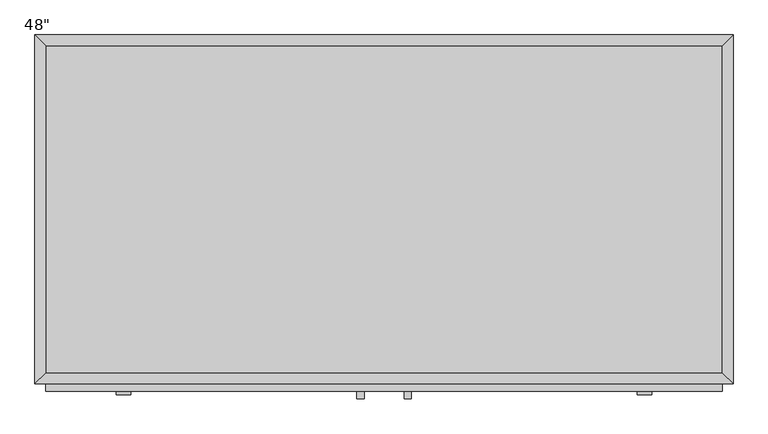
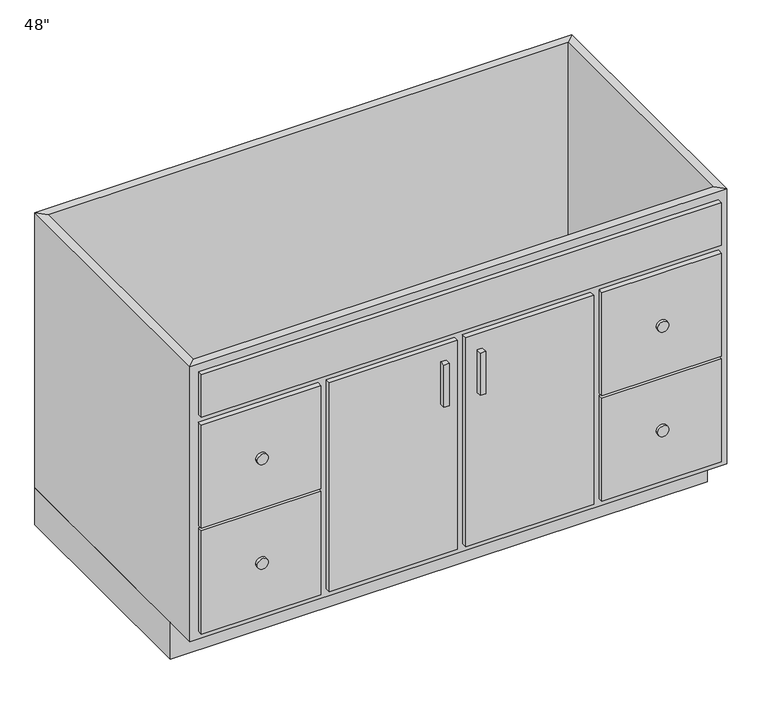
"""IFC4 building model written with IfcOpenShell, lengths in millimetres: furniture geometry."""

import ifcopenshell
import ifcopenshell.guid

model = None  # the IFC model being written
_history = None  # IfcOwnerHistory: only IFC2X3 demands one
_inside = {}  # id of a spatial element -> (the spatial element, [elements in it])
_under = {}  # id of a project, library or spatial element -> (it, [spatial elements below it])
_declared = {}  # id of a project -> (the project, [libraries it declares])
_typed = {}  # id of a type object -> (the type object, [elements of that type])
_made_of = {}  # id of a material, layer set ... -> (it, [elements and type objects made of it])


def new_model(schema):
    """Start an empty IFC model of exactly this schema.

    Asked for "IFC4X3", IfcOpenShell would pick the latest addendum, in which some entities
    have other attributes; the version numbers below select the first issue.
    IFC2X3 requires an IfcOwnerHistory on every rooted entity: one is made here for all.
    """
    global model, _history
    if schema == "IFC4X3":
        model = ifcopenshell.file(schema_version=(4, 3, 0, 0))
    else:
        model = ifcopenshell.file(schema=schema)
    _inside.clear()
    _under.clear()
    _declared.clear()
    _typed.clear()
    _made_of.clear()
    _history = None
    if model.schema == "IFC2X3":
        org = make("IfcOrganization", Name="unknown")
        user = make(
            "IfcPersonAndOrganization",
            ThePerson=make("IfcPerson", FamilyName="unknown"),
            TheOrganization=org,
        )
        app = make(
            "IfcApplication",
            ApplicationDeveloper=org,
            Version="unknown",
            ApplicationFullName="unknown",
            ApplicationIdentifier="unknown",
        )
        _history = make(
            "IfcOwnerHistory",
            OwningUser=user,
            OwningApplication=app,
            ChangeAction="ADDED",
            CreationDate=0,
        )
    return model


def make(cls, **values):
    """One entity of the class cls with the attributes given. An attribute that is None is left unset."""
    return model.create_entity(
        cls, **{name: value for name, value in values.items() if value is not None}
    )


def rooted(cls, **values):
    """An entity with a GlobalId (a new one), such as an element, a storey or a relation."""
    return make(cls, GlobalId=ifcopenshell.guid.new(), OwnerHistory=_history, **values)


def si_unit(unit_type, name, prefix=None):
    """IfcSIUnit, for example si_unit("LENGTHUNIT", "METRE", prefix="MILLI")."""
    return make("IfcSIUnit", UnitType=unit_type, Prefix=prefix, Name=name)


def assignment(units):
    """IfcUnitAssignment: the units of a project."""
    return None if units is None else make("IfcUnitAssignment", Units=units)


def point(xyz):
    """IfcCartesianPoint."""
    return None if xyz is None else make("IfcCartesianPoint", Coordinates=xyz)


def direction(xyz):
    """IfcDirection."""
    return None if xyz is None else make("IfcDirection", DirectionRatios=xyz)


def frame(location, z_axis=None, x_axis=None):
    """IfcAxis2Placement3D, a coordinate frame: its origin and axes. An axis left out is left unset."""
    return make(
        "IfcAxis2Placement3D",
        Location=point(location),
        Axis=direction(z_axis),
        RefDirection=direction(x_axis),
    )


def frame_2d(location, x_axis=None):
    """IfcAxis2Placement2D, a coordinate frame in the plane: its origin and x axis."""
    return make(
        "IfcAxis2Placement2D", Location=point(location), RefDirection=direction(x_axis)
    )


def origin():
    """The frame at (0, 0, 0) with its axes left unset."""
    return frame((0.0, 0.0, 0.0))


def origin_with_axes():
    """The frame at (0, 0, 0) with the z axis (0, 0, 1) and the x axis (1, 0, 0) written out."""
    return frame((0.0, 0.0, 0.0), z_axis=(0.0, 0.0, 1.0), x_axis=(1.0, 0.0, 0.0))


def place(relative_to, where):
    """IfcLocalPlacement: puts the frame where relative to a parent placement (None: the world)."""
    return make(
        "IfcLocalPlacement", PlacementRelTo=relative_to, RelativePlacement=where
    )


def context(
    kind, dimensions, precision=None, world=None, true_north=None, identifier=None
):
    """IfcGeometricRepresentationContext, for example the 3D "Model" context."""
    return make(
        "IfcGeometricRepresentationContext",
        ContextIdentifier=identifier,
        ContextType=kind,
        CoordinateSpaceDimension=dimensions,
        Precision=precision,
        WorldCoordinateSystem=world,
        TrueNorth=true_north,
    )


def project(units=None, contexts=None):
    """IfcProject with its units and contexts."""
    return rooted(
        "IfcProject",
        Name="project",
        RepresentationContexts=contexts,
        UnitsInContext=assignment(units),
    )


def spatial(cls, under=None, at=None, **own):
    """A site, building, storey or space (cls), placed at a placement, below another one or the project."""
    s = rooted(cls, ObjectPlacement=at, **own)
    if under is not None:
        _under.setdefault(under.id(), (under, []))[1].append(s)
    return s


def polyline(points):
    """IfcPolyline through the points."""
    return make("IfcPolyline", Points=[point(p) for p in points])


def circle_curve(where, radius):
    """IfcCircle in the frame where."""
    return make("IfcCircle", Position=where, Radius=radius)


def trimmed(basis, trim1, trim2, sense, master):
    """IfcTrimmedCurve: the piece of a basis curve between two trims."""
    return make(
        "IfcTrimmedCurve",
        BasisCurve=basis,
        Trim1=trim1,
        Trim2=trim2,
        SenseAgreement=sense,
        MasterRepresentation=master,
    )


def segment(curve, same_sense, transition):
    """IfcCompositeCurveSegment."""
    return make(
        "IfcCompositeCurveSegment",
        Transition=transition,
        SameSense=same_sense,
        ParentCurve=curve,
    )


def composite_curve(segments, self_intersect=None):
    """IfcCompositeCurve: segments joined end to end."""
    return make("IfcCompositeCurve", Segments=segments, SelfIntersect=self_intersect)


def outline(outer, holes=None, kind="AREA"):
    """IfcArbitraryClosedProfileDef: a profile drawn as a closed curve; with holes, ...WithVoids."""
    if holes is None:
        return make("IfcArbitraryClosedProfileDef", ProfileType=kind, OuterCurve=outer)
    return make(
        "IfcArbitraryProfileDefWithVoids",
        ProfileType=kind,
        OuterCurve=outer,
        InnerCurves=holes,
    )


def extrude(swept, where, along, depth):
    """IfcExtrudedAreaSolid: the profile swept, set in the frame where, extruded along a direction by depth."""
    return make(
        "IfcExtrudedAreaSolid",
        SweptArea=swept,
        Position=where,
        ExtrudedDirection=direction(along),
        Depth=depth,
    )


def faces_of(points, faces, orient=None, outer=None):
    """IfcFace entities. A face is a list of loops; a loop is a list of indices into points, from 0.

    orient and outer hold one flag for each loop. By default every Orientation is true, the
    first loop of a face is its IfcFaceOuterBound and the others are IfcFaceBound.
    """
    made = []
    for i, loops in enumerate(faces):
        bounds = []
        for j, loop in enumerate(loops):
            is_outer = j == 0 if outer is None else outer[i][j]
            bounds.append(
                make(
                    "IfcFaceOuterBound" if is_outer else "IfcFaceBound",
                    Bound=make("IfcPolyLoop", Polygon=[points[k] for k in loop]),
                    Orientation=True if orient is None else orient[i][j],
                )
            )
        made.append(make("IfcFace", Bounds=bounds))
    return made


def faceted_brep(points, faces, orient=None, outer=None, voids=None):
    """IfcFacetedBrep: a solid bounded by flat faces; with voids (closed shells), ...WithVoids."""
    shared = [point(p) for p in points]
    hull = make("IfcClosedShell", CfsFaces=faces_of(shared, faces, orient, outer))
    if voids is None:
        return make("IfcFacetedBrep", Outer=hull)
    return make(
        "IfcFacetedBrepWithVoids",
        Outer=hull,
        Voids=[
            make(cls, CfsFaces=faces_of(shared, fs, o, b)) for cls, fs, o, b in voids
        ],
    )


def shape(context_of_items, identifier, shape_type, items):
    """IfcShapeRepresentation: the items that make up one representation, for example the "Body"."""
    return make(
        "IfcShapeRepresentation",
        ContextOfItems=context_of_items,
        RepresentationIdentifier=identifier,
        RepresentationType=shape_type,
        Items=items,
    )


def source(mapping_origin, context_of_items, identifier, shape_type, items):
    """IfcRepresentationMap: a shape defined once, which mapped items show again and again."""
    return make(
        "IfcRepresentationMap",
        MappingOrigin=mapping_origin,
        MappedRepresentation=shape(context_of_items, identifier, shape_type, items),
    )


def transform(
    local_origin,
    x_axis=None,
    y_axis=None,
    z_axis=None,
    scale=None,
    scale2=None,
    scale3=None,
    uniform=True,
):
    """IfcCartesianTransformationOperator3D, or its non-uniform kind. x_axis, y_axis, z_axis: its Axis1, 2, 3."""
    if uniform:
        return make(
            "IfcCartesianTransformationOperator3D",
            Axis1=direction(x_axis),
            Axis2=direction(y_axis),
            LocalOrigin=point(local_origin),
            Scale=scale,
            Axis3=direction(z_axis),
        )
    return make(
        "IfcCartesianTransformationOperator3DnonUniform",
        Axis1=direction(x_axis),
        Axis2=direction(y_axis),
        LocalOrigin=point(local_origin),
        Scale=scale,
        Axis3=direction(z_axis),
        Scale2=scale2,
        Scale3=scale3,
    )


def mapped(mapping_source, mapping_target):
    """IfcMappedItem: shows the shape of a source again, moved by a transform."""
    return make(
        "IfcMappedItem", MappingSource=mapping_source, MappingTarget=mapping_target
    )


def made_of(thing, what):
    """Note that an element or type object is made of a material, layer set ...; save() writes the relation."""
    if what is not None:
        _made_of.setdefault(what.id(), (what, []))[1].append(thing)
    return thing


def element(
    cls,
    number,
    at=None,
    inside=None,
    cuts=None,
    type_object=None,
    material=None,
    context=None,
    identifier="Body",
    shape_type=None,
    held_by="IfcProductDefinitionShape",
    body=None,
    shapes=None,
    **own,
):
    """One element of the class cls, such as IfcWall. Its Tag is "e" and its number.

    at: its placement. inside: the storey or other place that contains it. cuts: it is an
    opening in that element (IfcRelVoidsElement). A single representation is given by context,
    identifier, shape_type and body (its items); several are given by shapes. held_by: the class
    of the entity that holds the representations. save() writes the other relations.
    """
    e = rooted(cls, Tag="e%d" % number, ObjectPlacement=at, **own)
    if body is not None:
        shapes = [shape(context, identifier, shape_type, body)]
    if shapes is not None:
        e.Representation = make(held_by, Representations=shapes)
    if inside is not None:
        _inside.setdefault(inside.id(), (inside, []))[1].append(e)
    if cuts is not None:
        rooted(
            "IfcRelVoidsElement", RelatingBuildingElement=cuts, RelatedOpeningElement=e
        )
    if type_object is not None:
        _typed.setdefault(type_object.id(), (type_object, []))[1].append(e)
    return made_of(e, material)


def aggregate(whole, parts):
    """IfcRelAggregates: a whole, such as a stair, and the parts it consists of."""
    return rooted("IfcRelAggregates", RelatingObject=whole, RelatedObjects=parts)


def save(model, path):
    """Write the relations noted so far, then the file.

    IfcRelAggregates (storeys below a building ...), IfcRelContainedInSpatialStructure (elements
    in a storey), IfcRelDefinesByType, IfcRelAssociatesMaterial and IfcRelDeclares: one each for
    every whole, place, type object, material and project.
    """
    for whole, parts in _under.values():
        aggregate(whole, parts)
    for where, things in _inside.values():
        rooted(
            "IfcRelContainedInSpatialStructure",
            RelatedElements=things,
            RelatingStructure=where,
        )
    for kind, things in _typed.values():
        rooted("IfcRelDefinesByType", RelatedObjects=things, RelatingType=kind)
    for what, things in _made_of.values():
        rooted("IfcRelAssociatesMaterial", RelatedObjects=things, RelatingMaterial=what)
    for by, libraries in _declared.values():
        rooted("IfcRelDeclares", RelatingContext=by, RelatedDefinitions=libraries)
    model.write(path)


def furniture_7e5e5cd5(model_context):
    return source(origin(), model_context, "Body", "SolidModel", [
        extrude(outline(polyline([(55.91996, -635.0), (43.21996, -635.0), (43.21996, -622.3), (55.91996, -622.3), (55.91996, -635.0)])), frame((0.0, 0.0, 469.9), z_axis=(0.0, 0.0, 1.0), x_axis=(1.0, 0.0, 0.0)), (0.0, 0.0, 1.0), 101.6),
        extrude(outline(polyline([(138.46996, -635.0), (125.76996, -635.0), (125.76996, -622.3), (138.46996, -622.3), (138.46996, -635.0)])), frame((0.0, 0.0, 469.9), z_axis=(0.0, 0.0, 1.0), x_axis=(1.0, 0.0, 0.0)), (0.0, 0.0, 1.0), 101.6),
        extrude(outline(composite_curve([segment(trimmed(circle_curve(frame_2d((484.1875, -363.97379)), 12.7), [point((484.1875, -376.67379))], [point((484.1875, -351.27379))], False, "CARTESIAN"), True, "CONTINUOUS"), segment(trimmed(circle_curve(frame_2d((484.1875, -363.97379)), 12.7), [point((484.1875, -351.27379))], [point((484.1875, -376.67379))], False, "CARTESIAN"), True, "CONTINUOUS")], self_intersect=False)), frame((0.0, -628.65, 0.0), z_axis=(0.0, 1.0, 0.0), x_axis=(0.0, 0.0, 1.0)), (0.0, 0.0, 1.0), 6.35),
        extrude(outline(composite_curve([segment(trimmed(circle_curve(frame_2d((233.3625, -363.97379)), 12.7), [point((233.3625, -376.67379))], [point((233.3625, -351.27379))], False, "CARTESIAN"), True, "CONTINUOUS"), segment(trimmed(circle_curve(frame_2d((233.3625, -363.97379)), 12.7), [point((233.3625, -351.27379))], [point((233.3625, -376.67379))], False, "CARTESIAN"), True, "CONTINUOUS")], self_intersect=False)), frame((0.0, -628.65, 0.0), z_axis=(0.0, 1.0, 0.0), x_axis=(0.0, 0.0, 1.0)), (0.0, 0.0, 1.0), 6.35),
        extrude(outline(composite_curve([segment(trimmed(circle_curve(frame_2d((233.3625, 545.66371)), 12.7), [point((233.3625, 532.96371))], [point((233.3625, 558.36371))], False, "CARTESIAN"), True, "CONTINUOUS"), segment(trimmed(circle_curve(frame_2d((233.3625, 545.66371)), 12.7), [point((233.3625, 558.36371))], [point((233.3625, 532.96371))], False, "CARTESIAN"), True, "CONTINUOUS")], self_intersect=False)), frame((0.0, -628.65, 0.0), z_axis=(0.0, 1.0, 0.0), x_axis=(0.0, 0.0, 1.0)), (0.0, 0.0, 1.0), 6.35),
        extrude(outline(composite_curve([segment(trimmed(circle_curve(frame_2d((484.1875, 545.66371)), 12.7), [point((484.1875, 532.96371))], [point((484.1875, 558.36371))], False, "CARTESIAN"), True, "CONTINUOUS"), segment(trimmed(circle_curve(frame_2d((484.1875, 545.66371)), 12.7), [point((484.1875, 558.36371))], [point((484.1875, 532.96371))], False, "CARTESIAN"), True, "CONTINUOUS")], self_intersect=False)), frame((0.0, -628.65, 0.0), z_axis=(0.0, 1.0, 0.0), x_axis=(0.0, 0.0, 1.0)), (0.0, 0.0, 1.0), 6.35),
        extrude(outline(polyline([(681.39496, -19.05), (681.39496, -590.55), (-499.70504, -590.55), (-499.70504, -19.05), (681.39496, -19.05)])), frame((0.0, 0.0, 88.9), z_axis=(0.0, 0.0, 1.0), x_axis=(1.0, 0.0, 0.0)), (0.0, 0.0, 1.0), 19.05),
        faceted_brep([(681.39496, -590.55, 749.3), (681.39496, -590.55, 88.9), (-499.70504, -590.55, 88.9), (-499.70504, -590.55, 749.3), (700.44496, -609.6, 749.3), (-518.75504, -609.6, 749.3), (700.44496, -609.6, 88.9), (-518.75504, -609.6, 88.9), (-499.70504, -19.05, 88.9), (-499.70504, -19.05, 749.3), (-518.75504, 0.0, 749.3), (-518.75504, 0.0, 88.9), (681.39496, -19.05, 88.9), (681.39496, -19.05, 749.3), (700.44496, 0.0, 749.3), (700.44496, 0.0, 88.9)], [[[0, 1, 2, 3]], [[4, 0, 3, 5]], [[6, 4, 5, 7]], [[1, 6, 7, 2]], [[3, 2, 8, 9]], [[5, 3, 9, 10]], [[7, 5, 10, 11]], [[2, 7, 11, 8]], [[9, 8, 12, 13]], [[10, 9, 13, 14]], [[11, 10, 14, 15]], [[8, 11, 15, 12]], [[13, 12, 1, 0]], [[14, 13, 0, 4]], [[15, 14, 4, 6]], [[12, 15, 6, 1]]]),
        extrude(outline(polyline([(700.44496, 0.0), (700.44496, -533.4), (-518.75504, -533.4), (-518.75504, 0.0), (700.44496, 0.0)])), origin_with_axes(), (0.0, 0.0, 1.0), 88.9),
        extrude(outline(polyline([(681.39496, -622.3), (-499.70504, -622.3), (-499.70504, -609.6), (681.39496, -609.6), (681.39496, -622.3)])), frame((0.0, 0.0, 628.65), z_axis=(0.0, 0.0, 1.0), x_axis=(1.0, 0.0, 0.0)), (0.0, 0.0, 1.0), 101.6),
        extrude(outline(polyline([(681.39496, -622.3), (409.93246, -622.3), (409.93246, -609.6), (681.39496, -609.6), (681.39496, -622.3)])), frame((0.0, 0.0, 361.95), z_axis=(0.0, 0.0, 1.0), x_axis=(1.0, 0.0, 0.0)), (0.0, 0.0, 1.0), 247.65),
        extrude(outline(polyline([(681.39496, -622.3), (409.93246, -622.3), (409.93246, -609.6), (681.39496, -609.6), (681.39496, -622.3)])), frame((0.0, 0.0, 107.95), z_axis=(0.0, 0.0, 1.0), x_axis=(1.0, 0.0, 0.0)), (0.0, 0.0, 1.0), 247.65),
        extrude(outline(polyline([(-228.24254, -622.3), (-499.70504, -622.3), (-499.70504, -609.6), (-228.24254, -609.6), (-228.24254, -622.3)])), frame((0.0, 0.0, 361.95), z_axis=(0.0, 0.0, 1.0), x_axis=(1.0, 0.0, 0.0)), (0.0, 0.0, 1.0), 247.65),
        extrude(outline(polyline([(-228.24254, -622.3), (-499.70504, -622.3), (-499.70504, -609.6), (-228.24254, -609.6), (-228.24254, -622.3)])), frame((0.0, 0.0, 107.95), z_axis=(0.0, 0.0, 1.0), x_axis=(1.0, 0.0, 0.0)), (0.0, 0.0, 1.0), 247.65),
        extrude(outline(polyline([(81.31996, -622.3), (-209.19254, -622.3), (-209.19254, -609.6), (81.31996, -609.6), (81.31996, -622.3)])), frame((0.0, 0.0, 107.95), z_axis=(0.0, 0.0, 1.0), x_axis=(1.0, 0.0, 0.0)), (0.0, 0.0, 1.0), 501.65),
        extrude(outline(polyline([(390.88246, -622.3), (100.36996, -622.3), (100.36996, -609.6), (390.88246, -609.6), (390.88246, -622.3)])), frame((0.0, 0.0, 107.95), z_axis=(0.0, 0.0, 1.0), x_axis=(1.0, 0.0, 0.0)), (0.0, 0.0, 1.0), 501.65),
    ])


if __name__ == "__main__":
    model = new_model("IFC4")
    model_context = context("Model", 3, world=origin())
    ifc_project = project(units=[si_unit("LENGTHUNIT", "METRE", prefix="MILLI")], contexts=[model_context])
    site = spatial("IfcSite", under=ifc_project)
    building = spatial("IfcBuilding", under=site)
    placement = place(None, origin())
    furniture_shape = furniture_7e5e5cd5(model_context)
    element("IfcFurniture", 1, ObjectType="Vanity Cabinet-Double Door & 4 Drawer : 48\"", at=placement, inside=building, context=model_context, shape_type="MappedRepresentation", body=[
        mapped(furniture_shape, transform((0.0, 0.0, 0.0), x_axis=(1.0, 0.0, 0.0), y_axis=(0.0, 1.0, 0.0), z_axis=(0.0, 0.0, 1.0))),
    ])
    save(model, "model.ifc")

# Revit data of these elements
# Type "Vanity Cabinet-Double Door & 4 Drawer : 48\""
#   Assembly Code = "C1030410"
#   Depth = 2' - 0"
#   Height = 2' - 5 1/2"
#   Toe Depth = 0' - 3"
#   Toe Height = 0' - 3 1/2"
#   Width = 4' - 0"
#   Cabinet Material = Cherry
#   Door/Drawer Material = Cherry
#   Handle Material = Steel, Chrome Plated
#   Default Elevation = 0
# Element 1 (IfcFurniture, "Vanity Cabinet-Double Door & 4 Drawer : 48\"")
#   Materials on its faces: "Cherry", "Steel, Chrome Plated", "Cabinets"
# Materials
#   "Cherry": class "Wood", colour RGB 157 77 38, transparency 0, Description = "Prunus Serotina", Cost = 0
#   "Steel, Chrome Plated": class "Metal", colour RGB 120 120 120, transparency 0, Description = "Chromiuim plated steel", Cost = 0
#   "Cabinets": class "Unassigned", colour RGB 249 249 249, transparency 0
